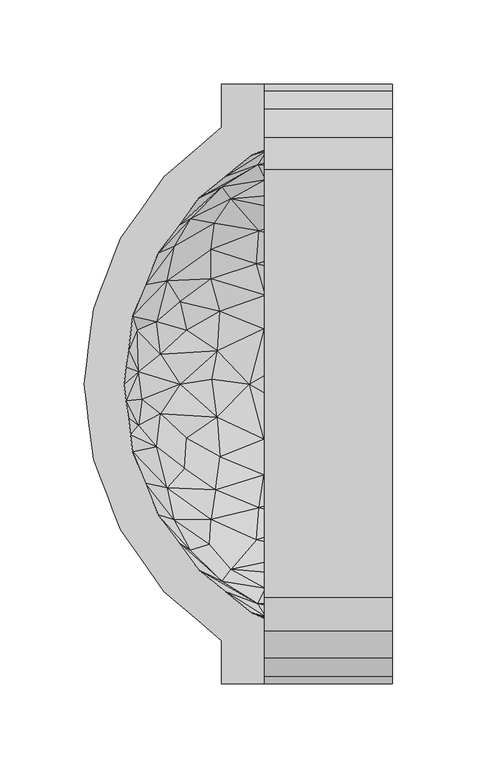
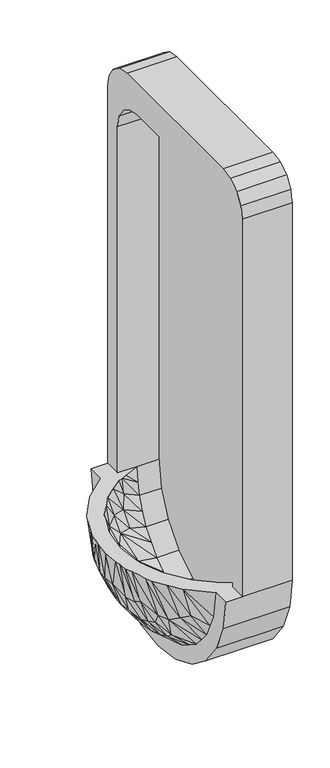
"""IFC4 building model written with IfcOpenShell, lengths in millimetres: proxy geometry, Urinal-Wall-3D:Urinal-Wall-3D:2445:Urinal-Wall-3D:2445 : Urinal-Wall-3D:Urinal-Wall-3D:2445:300497 : Urinal-Wall-3D:Urinal-Wall-3D:2445:Urinal-Wall-3D:2445 : Urinal-Wall-3D:Urinal-Wall-3D:2445:300497."""

from ifc_helpers import new_model, si_unit, origin, place, context, project, spatial, triangles, source, transform, mapped, element, save


def generic_models_a574338b(model_context):
    return source(origin(), model_context, "Body", "Tessellation", [
        triangles([(647621.4931641, -572395.2011719, 609.6), (647612.1914062, -572368.1144531, 609.6), (647599.2433594, -572386.4575195, 609.6), (647595.1505859, -572396.9499023, 609.6), (647645.0824219, -572332.5817383, 609.6), (647625.0650391, -572349.7713867, 609.6), (647645.5289063, -572362.6450195, 609.6), (647633.4738281, -572378.9044922, 609.6), (647613.9029297, -572413.9907227, 609.6), (647587.1138672, -572417.8602539, 609.6), (647606.3871094, -572432.7430664, 609.6), (647591.1322266, -572407.4050781, 609.6), (647581.6816406, -572439.4775391, 609.6), (647583.0210938, -572428.3526367, 609.6), (647603.8570313, -572452.8348633, 609.6), (647580.2677734, -572450.6024414, 609.6), (647602.5175781, -572462.8435547, 609.6), (647578.9283203, -572461.7645508, 609.6), (647684.521875, -572295.0770508, 609.6), (647659.1466797, -572295.0770508, 609.6), (647684.521875, -572320.4894531, 609.6), (647659.1466797, -572320.4894531, 609.6), (647677.0060547, -572337.1954102, 609.6), (647661.2302734, -572349.9202148, 609.6), (647713.8410156, -572320.4894531, 609.6), (647690.8470703, -572330.9446289, 609.6), (647683.9265625, -572334.0700195, 609.6), (647605.1220703, -572442.7889648, 609.6), (647601.2525391, -572472.8894531, 609.6), (647577.5144531, -572472.8894531, 609.6), (647578.9283203, -572484.0143555, 609.6), (647580.2677734, -572495.1764648, 609.6), (647602.5175781, -572482.9353516, 609.6), (647603.8570313, -572492.944043, 609.6), (647605.1220703, -572502.9899414, 609.6), (647581.6816406, -572506.3013672, 609.6), (647606.3871094, -572513.0358398, 609.6), (647583.0210938, -572517.4262695, 609.6), (647587.1138672, -572527.9186523, 609.6), (647613.9029297, -572531.8253906, 609.6), (647591.1322266, -572538.3738281, 609.6), (647595.1505859, -572548.8662109, 609.6), (647621.4931641, -572550.5777344, 609.6), (647599.2433594, -572559.3213867, 609.6), (647612.1914062, -572577.6644531, 609.6), (647633.4738281, -572566.8744141, 609.6), (647645.5289063, -572583.1338867, 609.6), (647625.0650391, -572596.0075195, 609.6), (647661.2302734, -572595.8586914, 609.6), (647645.0824219, -572613.197168, 609.6), (647690.8470703, -572614.8342773, 609.6), (647677.0060547, -572608.5834961, 609.6), (647684.521875, -572625.2894531, 609.6), (647659.1466797, -572625.2894531, 609.6), (647659.1466797, -572650.7018555, 609.6), (647702.3068359, -572620.0804687, 609.6), (647713.8410156, -572625.2894531, 609.6), (647684.521875, -572650.7018555, 609.6), (647685.8613281, -572334.4420898, 583.9469873), (647659.2955078, -572589.8683594, 571.4722764), (647713.8410156, -572391.3316406, 482.6979349), (647713.8410156, -572373.1001953, 494.4237817), (647681.3220703, -572381.9182617, 505.4282335), (647664.8765625, -572582.7618164, 545.0935813), (647685.1171875, -572594.184375, 538.9458097), (647713.8410156, -572586.8917969, 510.8150414), (647609.8101563, -572465.6712891, 558.6713862), (647664.8765625, -572363.0170898, 545.0936176), (647713.8410156, -572358.8871094, 510.8150414), (647685.1171875, -572351.5945313, 538.9458097), (647713.8410156, -572554.4472656, 482.6979349), (647679.8337891, -572565.3117188, 507.9383274), (647713.8410156, -572572.6787109, 494.4237817), (647684.4474609, -572440.1472656, 473.4506433), (647685.3404297, -572420.0182617, 479.4091822), (647658.1792969, -572429.7292969, 495.410422), (647656.6166016, -572453.2069336, 490.4112722), (647675.5921875, -572472.8894531, 474.7844645), (647713.8410156, -572326.6658203, 566.663958), (647713.8410156, -572323.8380859, 586.2369638), (647680.6523438, -572342.5904297, 564.4870923), (647659.2955078, -572355.9105469, 571.4722764), (647638.3851562, -572440.9658203, 512.4167241), (647622.9070313, -572455.2533203, 531.3763953), (647638.3851562, -572504.8875, 512.4541128), (647622.9070313, -572490.3767578, 531.3513605), (647620.6746094, -572509.9848633, 543.0548249), (647679.8337891, -572401.4519531, 492.2453536), (647658.1792969, -572516.0496094, 495.410422), (647684.4474609, -572526.5791992, 480.2694131), (647684.3730469, -572505.5572266, 473.4754601), (647630.7949219, -572553.4426758, 564.2788201), (647626.7021484, -572534.3182617, 548.7818009), (647640.8408203, -572374.8117188, 571.7064554), (647637.1945313, -572522.8584961, 522.0602489), (647685.8613281, -572611.3368164, 583.9469873), (647680.6523438, -572603.1884766, 564.4870923), (647713.8410156, -572344.6740234, 527.2063374), (647713.8410156, -572335.6699219, 546.9351477), (647652.0773438, -572568.027832, 542.0659318), (647655.0539063, -572377.3045898, 538.0613434), (647652.7470703, -572392.8199219, 523.79539), (647713.8410156, -572610.1089844, 546.9351477), (647681.3220703, -572546.1500977, 492.3042526), (647713.8410156, -572536.2158203, 470.9720881), (647609.8845703, -572497.2600586, 563.910783), (647608.9916016, -572440.9658203, 572.3650998), (647631.1669922, -572391.2200195, 565.2611003), (647626.7021484, -572411.4606445, 548.7818009), (647713.8410156, -572619.1130859, 566.663958), (647713.8410156, -572623.6151367, 597.9184819), (647713.8410156, -572621.9408203, 586.2369638), (647713.8410156, -572409.600293, 470.9720881), (647640.5431641, -572571.4136719, 573.9630401), (647655.4259766, -572535.7321289, 507.6571309), (647713.8410156, -572451.1977539, 458.7512135), (647713.8410156, -572472.8894531, 458.7512135), (647713.8410156, -572494.5811523, 458.7512135), (647713.8410156, -572601.1048828, 527.2063374), (647620.6746094, -572435.794043, 543.0548249), (647713.8410156, -572430.3990234, 464.8616326), (647611.89375, -572481.9679688, 553.1137676), (647634.4412109, -572472.8894531, 512.2263288), (647656.4677734, -572492.5347656, 490.5842631), (647634.5900391, -572423.887793, 525.2664122), (647652.7470703, -572552.9589844, 523.79539), (647652.7470703, -572410.4188477, 510.2499232), (647653.3423828, -572469.9873047, 491.7342293), (647713.8410156, -572515.3798828, 464.8616326), (647747.9970703, -572326.6658203, 566.663958), (647747.9970703, -572320.4894531, 609.6), (647747.9970703, -572344.6740234, 527.2063374), (647747.9970703, -572409.600293, 470.9720881), (647747.9970703, -572373.1001953, 494.4237817), (647747.9970703, -572451.1977539, 458.7512135), (647747.9970703, -572494.5811523, 458.7512135), (647747.9970703, -572536.2158203, 470.9720881), (647747.9970703, -572572.6787109, 494.4237817), (647747.9970703, -572625.2894531, 609.6), (647747.9970703, -572619.1130859, 566.663958), (647747.9970703, -572601.1048828, 527.2063374), (647760.721875, -572609.625293, 1268.066494), (647760.721875, -572619.3363281, 1266.1330364), (647760.721875, -572627.559082, 1260.6271225), (647760.721875, -572648.7670898, 1228.9201916), (647760.721875, -572599.8770508, 1269.9999516), (647760.721875, -572641.3256836, 1246.8807232), (647760.721875, -572635.819043, 1255.1210632), (647760.721875, -572295.0770508, 1219.2), (647760.721875, -572345.9018555, 1269.9999516), (647760.721875, -572318.2198242, 1260.6271225), (647760.721875, -572336.1536133, 1268.066494), (647760.721875, -572304.4532227, 1246.8807232), (647760.721875, -572326.4425781, 1266.1330364), (647760.721875, -572297.0118164, 1228.9201916), (647760.721875, -572309.9598633, 1255.1210632), (647760.721875, -572298.946582, 1238.6403831), (647760.721875, -572646.8323242, 1238.6403831), (647760.721875, -572650.7018555, 1219.2), (647760.721875, -572644.6371094, 563.5819877), (647760.721875, -572295.0770508, 609.6), (647760.721875, -572650.7018555, 609.6), (647760.721875, -572318.9267578, 520.7000121), (647760.721875, -572626.8521484, 520.7000121), (647760.721875, -572598.6120117, 483.876424), (647760.721875, -572561.7770508, 455.6206996), (647760.721875, -572347.1668945, 483.876424), (647760.721875, -572301.1417969, 563.5819877), (647760.721875, -572518.9145508, 437.8583754), (647760.721875, -572384.0018555, 455.6206996), (647760.721875, -572426.8643555, 437.8583754), (647760.721875, -572472.8894531, 431.7999879), (647659.1466797, -572301.1417969, 563.5819877), (647659.1466797, -572347.1668945, 483.876424), (647659.1466797, -572318.9267578, 520.7000121), (647659.1466797, -572384.0018555, 455.6206996), (647659.1466797, -572426.8643555, 437.8583754), (647659.1466797, -572472.8894531, 431.7999879), (647659.1466797, -572518.9145508, 437.8583754), (647659.1466797, -572561.7770508, 455.6206996), (647659.1466797, -572626.8521484, 520.7000121), (647659.1466797, -572644.6371094, 563.5819877), (647659.1466797, -572598.6120117, 483.876424), (647659.1466797, -572472.8894531, 458.7512135), (647659.1466797, -572494.5811523, 458.7512135), (647659.1466797, -572451.1977539, 458.7512135), (647659.1466797, -572554.4472656, 482.6979349), (647659.1466797, -572536.2158203, 470.9720881), (647659.1466797, -572572.6787109, 494.4237817), (647659.1466797, -572515.3798828, 464.8616326), (647659.1466797, -572430.3990234, 464.8616326), (647659.1466797, -572409.600293, 470.9720881), (647659.1466797, -572391.3316406, 482.6979349), (647659.1466797, -572373.1001953, 494.4237817), (647659.1466797, -572358.8871094, 510.8150414), (647659.1466797, -572344.6740234, 527.2063374), (647659.1466797, -572610.1089844, 546.9351477), (647659.1466797, -572601.1048828, 527.2063374), (647659.1466797, -572586.8917969, 510.8150414), (647659.1466797, -572622.2384766, 588.2859303), (647659.1466797, -572619.1130859, 566.663958), (647659.1466797, -572335.6699219, 546.9351477), (647659.1466797, -572326.6658203, 566.663958), (647659.1466797, -572323.5404297, 588.2859303), (647636.5248047, -572400.1869141, 496.2975772), (647629.2322266, -572417.971875, 494.5229762), (647612.3402344, -572400.6333984, 530.1853706), (647635.7806641, -572346.7204102, 564.7131323), (647606.6847656, -572415.1069336, 529.1428834), (647627.5207031, -572385.5645508, 519.1144621), (647604.6011719, -572392.3734375, 557.7764917), (647618.7398438, -572375.3326172, 547.3545261), (647626.8509766, -572359.4080078, 557.2311399), (647630.94375, -572505.4828125, 484.5077808), (647630.94375, -572440.2960938, 484.5077808), (647594.9273438, -572409.7863281, 563.8420009), (647606.9080078, -572449.9699219, 512.8612101), (647585.4767578, -572457.7833984, 558.5052627), (647589.4951172, -572439.4775391, 553.8611421), (647626.8509766, -572586.3708984, 557.2311399), (647635.7806641, -572599.0584961, 564.7131323), (647630.94375, -572526.1699219, 491.8173274), (647607.9498047, -572515.3054688, 517.92133), (647612.3402344, -572545.1455078, 530.1853706), (647633.1761719, -572541.1643555, 497.2734624), (647631.6134766, -572554.89375, 508.7941981), (647592.9925781, -572524.4956055, 557.1740939), (647589.1230469, -572508.1245117, 555.9720234), (647625.7347656, -572485.5398438, 486.402905), (647600.8804688, -572494.9160156, 522.8274985), (647602.0710938, -572472.8894531, 518.0100964), (647627.7439453, -572462.6947266, 484.0731417), (647583.7652344, -572482.5632813, 563.1875713), (647607.9498047, -572430.4734375, 517.92133), (647590.4625, -572422.4367188, 564.5393057), (647609.4380859, -572556.9029297, 549.5402212), (647594.8529297, -572536.1786133, 564.3948741), (647618.7398438, -572570.4462891, 547.3544898), (647609.8845703, -572529.9650391, 522.8140182), (647684.521875, -572625.2894531, 1168.3999758), (647684.521875, -572623.6151367, 1176.8655928), (647684.521875, -572650.7018555, 1219.2), (647684.521875, -572621.4199219, 1187.8402863), (647684.521875, -572610.4066406, 1204.321039), (647684.521875, -572615.9132813, 1196.080699), (647684.521875, -572627.559082, 1260.6271225), (647684.521875, -572593.9239258, 1215.3330849), (647684.521875, -572602.1838867, 1209.8270256), (647684.521875, -572584.2128906, 1217.2665424), (647684.521875, -572599.8770508, 1269.9999516), (647684.521875, -572641.3256836, 1246.8807232), (647684.521875, -572322.4242187, 1178.1201674), (647684.521875, -572324.3589844, 1187.8402863), (647684.521875, -572295.0770508, 1219.2), (647684.521875, -572320.4894531, 1168.3999758), (647684.521875, -572351.8549805, 1215.3330849), (647684.521875, -572362.8310547, 1217.5160912), (647684.521875, -572345.9018555, 1269.9999516), (647684.521875, -572304.4532227, 1246.8807232), (647684.521875, -572335.3722656, 1204.321039), (647684.521875, -572343.5950195, 1209.8270256), (647684.521875, -572329.865625, 1196.080699), (647684.521875, -572318.2198242, 1260.6271225), (647684.521875, -572648.7670898, 1228.9201916), (647684.521875, -572646.8323242, 1238.6403831), (647684.521875, -572619.3363281, 1266.1330364), (647684.521875, -572606.9463867, 1268.5966942), (647684.521875, -572574.5018555, 1219.2), (647684.521875, -572635.819043, 1255.1210632), (647684.521875, -572371.2770508, 1219.2), (647684.521875, -572298.946582, 1238.6403831), (647684.521875, -572296.490918, 1226.2546566), (647684.521875, -572336.1536133, 1268.066494), (647684.521875, -572309.9598633, 1255.1210632), (647684.521875, -572326.4425781, 1266.1330364), (647747.9970703, -572320.4894531, 1168.3999758), (647747.9970703, -572324.3589844, 1187.8402863), (647747.9970703, -572322.1637695, 1176.8655928), (647747.9970703, -572335.3722656, 1204.321039), (647747.9970703, -572329.865625, 1196.080699), (647747.9970703, -572351.8549805, 1215.3330849), (647747.9970703, -572361.5660156, 1217.2665424), (647747.9970703, -572371.2770508, 1219.2), (647747.9970703, -572343.5950195, 1209.8270256), (647747.9970703, -572574.5018555, 1219.2), (647747.9970703, -572593.9239258, 1215.3330849), (647747.9970703, -572582.9478516, 1217.5160912), (647747.9970703, -572610.4066406, 1204.321039), (647747.9970703, -572602.1838867, 1209.8270256), (647747.9970703, -572621.4199219, 1187.8402863), (647747.9970703, -572623.3546875, 1178.1201674), (647747.9970703, -572625.2894531, 1168.3999758), (647747.9970703, -572615.9132813, 1196.080699)], [[1, 2, 3], [1, 3, 4], [5, 6, 7], [2, 8, 6], [1, 8, 2], [4, 9, 1], [9, 10, 11], [9, 12, 10], [13, 11, 14], [10, 14, 11], [15, 13, 16], [17, 16, 18], [12, 9, 4], [19, 20, 21], [21, 20, 22], [23, 22, 24], [21, 22, 23], [25, 21, 26], [27, 26, 21], [21, 23, 27], [7, 6, 8], [15, 28, 13], [11, 13, 28], [24, 22, 5], [17, 15, 16], [17, 18, 29], [24, 5, 7], [18, 30, 29], [31, 32, 33], [31, 33, 29], [33, 32, 34], [36, 35, 34], [35, 36, 37], [36, 34, 32], [31, 29, 30], [38, 39, 37], [37, 39, 40], [40, 41, 42], [39, 41, 40], [40, 42, 43], [43, 42, 44], [38, 37, 36], [43, 45, 46], [45, 43, 44], [47, 46, 48], [49, 47, 50], [51, 52, 53], [49, 54, 52], [45, 48, 46], [49, 50, 54], [54, 55, 53], [54, 53, 52], [57, 56, 53], [58, 53, 55], [56, 51, 53], [50, 47, 48], [59, 23, 24], [46, 47, 60], [61, 62, 63], [64, 65, 66], [29, 67, 17], [15, 17, 67], [68, 69, 70], [71, 72, 73], [74, 75, 76], [74, 77, 78], [79, 80, 27], [80, 26, 27], [25, 26, 80], [70, 81, 82], [7, 81, 24], [77, 83, 84], [85, 86, 87], [61, 63, 88], [89, 90, 91], [40, 92, 93], [94, 8, 1], [89, 85, 95], [96, 49, 52], [97, 60, 47], [7, 82, 81], [81, 98, 99], [72, 100, 64], [63, 101, 102], [96, 103, 97], [71, 104, 72], [71, 105, 104], [86, 106, 87], [15, 107, 28], [11, 28, 107], [108, 109, 102], [52, 110, 96], [56, 57, 111], [51, 56, 112], [52, 112, 110], [52, 51, 112], [112, 56, 111], [113, 61, 88], [64, 100, 114], [90, 89, 115], [79, 27, 59], [116, 78, 117], [118, 117, 78], [47, 49, 97], [8, 94, 82], [60, 65, 64], [8, 82, 7], [70, 82, 68], [119, 65, 97], [81, 70, 98], [62, 69, 68], [69, 98, 70], [114, 60, 64], [60, 97, 65], [64, 66, 73], [65, 119, 66], [109, 11, 120], [59, 99, 79], [97, 103, 119], [121, 75, 74], [33, 106, 122], [84, 83, 120], [87, 106, 35], [123, 122, 86], [85, 89, 124], [120, 83, 125], [92, 43, 114], [102, 101, 108], [109, 9, 11], [93, 126, 115], [93, 37, 40], [24, 81, 59], [99, 59, 81], [103, 96, 110], [97, 49, 96], [59, 27, 23], [74, 116, 121], [91, 124, 89], [102, 88, 63], [62, 68, 63], [68, 101, 63], [102, 127, 88], [127, 76, 75], [68, 94, 101], [108, 1, 9], [108, 101, 94], [109, 108, 9], [127, 102, 109], [125, 109, 120], [77, 74, 76], [88, 75, 113], [78, 116, 74], [83, 77, 76], [128, 78, 77], [113, 75, 121], [75, 88, 127], [94, 68, 82], [108, 94, 1], [76, 127, 125], [107, 84, 120], [67, 123, 84], [77, 84, 123], [76, 125, 83], [127, 109, 125], [104, 115, 126], [104, 105, 90], [104, 126, 72], [100, 72, 126], [64, 73, 72], [92, 100, 126], [100, 92, 114], [93, 92, 126], [40, 43, 92], [91, 129, 118], [129, 91, 90], [118, 78, 91], [124, 91, 78], [128, 124, 78], [86, 85, 124], [90, 105, 129], [90, 115, 104], [115, 89, 95], [43, 46, 114], [60, 114, 46], [86, 124, 123], [95, 87, 93], [67, 122, 123], [33, 34, 106], [35, 106, 34], [87, 95, 85], [115, 95, 93], [86, 122, 106], [35, 37, 87], [67, 29, 33], [37, 93, 87], [33, 122, 67], [107, 67, 84], [77, 123, 128], [11, 107, 120], [15, 67, 107], [124, 128, 123], [79, 130, 80], [80, 131, 25], [131, 80, 130], [132, 130, 99], [79, 99, 130], [99, 98, 132], [113, 133, 61], [61, 134, 62], [134, 61, 133], [62, 134, 69], [69, 132, 98], [132, 69, 134], [116, 135, 121], [121, 133, 113], [133, 121, 135], [135, 116, 117], [117, 118, 136], [117, 136, 135], [137, 105, 71], [71, 73, 138], [71, 138, 137], [136, 118, 129], [129, 105, 137], [129, 137, 136], [111, 57, 139], [112, 139, 140], [139, 112, 111], [112, 140, 110], [103, 140, 141], [140, 103, 110], [103, 141, 119], [66, 141, 138], [141, 66, 119], [66, 138, 73], [142, 143, 144], [145, 146, 142], [142, 147, 145], [144, 148, 147], [142, 144, 147], [149, 150, 146], [153, 151, 152], [151, 154, 152], [155, 152, 150], [153, 156, 151], [155, 157, 153], [152, 155, 153], [149, 155, 150], [145, 147, 158], [149, 146, 159], [162, 160, 161], [149, 159, 162], [163, 164, 165], [165, 166, 167], [160, 164, 168], [166, 169, 170], [164, 163, 168], [160, 168, 161], [161, 149, 162], [169, 171, 170], [167, 166, 170], [165, 167, 163], [171, 169, 172], [159, 146, 145], [19, 168, 173], [168, 19, 161], [19, 173, 20], [174, 175, 167], [163, 167, 175], [176, 174, 170], [167, 170, 174], [173, 168, 163], [163, 175, 173], [177, 176, 171], [170, 171, 176], [178, 177, 172], [171, 172, 177], [169, 179, 172], [178, 172, 179], [169, 166, 180], [180, 179, 169], [181, 164, 182], [160, 182, 164], [164, 181, 165], [183, 165, 181], [165, 183, 166], [180, 166, 183], [160, 162, 58], [58, 55, 182], [58, 182, 160], [184, 178, 185], [184, 186, 178], [178, 179, 185], [178, 186, 177], [180, 187, 188], [189, 187, 180], [190, 185, 179], [179, 188, 190], [179, 180, 188], [177, 191, 192], [191, 177, 186], [176, 192, 193], [192, 176, 177], [194, 174, 176], [174, 195, 175], [195, 174, 194], [195, 196, 175], [194, 176, 193], [181, 197, 198], [197, 181, 182], [199, 181, 198], [181, 199, 183], [182, 55, 200], [182, 200, 201], [200, 55, 54], [182, 201, 197], [199, 189, 183], [202, 173, 175], [203, 204, 173], [204, 20, 173], [20, 204, 22], [202, 203, 173], [202, 175, 196], [189, 180, 183], [6, 5, 204], [6, 204, 203], [22, 204, 5], [205, 206, 207], [208, 202, 196], [206, 209, 207], [210, 211, 212], [3, 2, 213], [214, 185, 190], [6, 202, 208], [191, 215, 206], [213, 212, 3], [6, 203, 202], [205, 207, 210], [211, 216, 10], [217, 218, 219], [220, 221, 45], [197, 201, 48], [214, 222, 223], [201, 200, 48], [200, 50, 48], [54, 50, 200], [2, 208, 213], [224, 225, 226], [227, 36, 228], [229, 230, 231], [198, 197, 221], [205, 193, 192], [221, 48, 45], [232, 229, 231], [221, 220, 198], [233, 231, 230], [219, 218, 16], [215, 217, 234], [234, 235, 209], [217, 215, 232], [224, 236, 237], [227, 237, 38], [189, 238, 226], [208, 196, 213], [2, 6, 208], [212, 195, 194], [195, 212, 213], [193, 210, 194], [212, 211, 4], [213, 196, 195], [48, 221, 197], [220, 45, 44], [238, 220, 44], [238, 199, 220], [236, 42, 41], [236, 41, 39], [187, 226, 225], [189, 199, 238], [199, 198, 220], [226, 236, 224], [206, 205, 192], [210, 207, 211], [215, 234, 206], [206, 234, 209], [194, 210, 212], [193, 205, 210], [206, 192, 191], [232, 215, 186], [191, 186, 215], [229, 184, 185], [184, 229, 232], [232, 231, 217], [217, 231, 218], [233, 218, 231], [16, 218, 18], [30, 18, 218], [229, 185, 214], [214, 230, 229], [223, 228, 230], [30, 233, 31], [32, 31, 233], [233, 230, 228], [218, 233, 30], [232, 186, 184], [227, 228, 223], [32, 233, 228], [223, 222, 239], [228, 36, 32], [227, 38, 36], [190, 188, 222], [188, 225, 222], [223, 239, 227], [222, 214, 190], [214, 223, 230], [234, 219, 235], [216, 207, 209], [219, 16, 13], [10, 12, 211], [12, 4, 211], [216, 14, 10], [216, 211, 207], [238, 44, 42], [239, 237, 227], [187, 225, 188], [236, 39, 237], [237, 39, 38], [239, 225, 224], [189, 226, 187], [236, 226, 238], [42, 236, 238], [216, 235, 14], [217, 219, 234], [13, 14, 235], [209, 235, 216], [219, 13, 235], [225, 239, 222], [237, 239, 224], [4, 3, 212], [53, 58, 240], [242, 241, 240], [242, 243, 241], [58, 242, 240], [242, 244, 245], [246, 247, 248], [249, 247, 250], [248, 244, 251], [245, 243, 242], [252, 253, 254], [19, 21, 255], [19, 255, 254], [255, 252, 254], [256, 257, 258], [259, 260, 261], [253, 262, 254], [261, 256, 263], [254, 262, 260], [251, 244, 264], [246, 248, 251], [251, 264, 265], [266, 247, 246], [264, 244, 242], [250, 247, 267], [268, 249, 250], [266, 267, 247], [251, 269, 246], [270, 268, 250], [259, 271, 260], [261, 263, 259], [272, 254, 260], [260, 271, 272], [258, 257, 270], [256, 273, 263], [263, 274, 259], [273, 275, 263], [256, 258, 273], [258, 270, 250], [276, 255, 25], [21, 25, 255], [25, 131, 276], [277, 253, 252], [277, 252, 278], [278, 255, 276], [255, 278, 252], [279, 260, 262], [279, 262, 280], [262, 277, 280], [277, 262, 253], [256, 281, 282], [256, 282, 257], [257, 283, 270], [283, 257, 282], [260, 279, 284], [260, 284, 261], [284, 256, 261], [256, 284, 281], [285, 268, 270], [270, 283, 285], [286, 247, 249], [286, 249, 287], [287, 268, 285], [268, 287, 249], [288, 244, 248], [288, 248, 289], [248, 286, 289], [286, 248, 247], [243, 290, 291], [243, 291, 241], [241, 292, 240], [292, 241, 291], [244, 288, 293], [244, 293, 245], [293, 243, 245], [243, 293, 290], [57, 240, 292], [240, 57, 53], [57, 292, 139], [159, 242, 162], [58, 162, 242], [148, 269, 251], [148, 251, 147], [251, 158, 147], [158, 251, 265], [242, 159, 145], [242, 145, 264], [145, 265, 264], [265, 145, 158], [146, 250, 267], [146, 267, 142], [142, 266, 143], [266, 142, 267], [246, 269, 148], [266, 246, 143], [148, 144, 246], [144, 143, 246], [150, 258, 250], [250, 146, 150], [156, 274, 263], [156, 263, 151], [263, 154, 151], [154, 263, 275], [258, 150, 152], [258, 152, 273], [152, 275, 273], [275, 152, 154], [149, 254, 272], [149, 272, 155], [155, 271, 157], [271, 155, 272], [259, 274, 156], [271, 259, 157], [156, 153, 259], [153, 157, 259], [161, 19, 149], [254, 149, 19], [292, 285, 276], [283, 282, 278], [282, 284, 280], [284, 279, 280], [284, 282, 281], [285, 283, 276], [293, 288, 289], [291, 290, 293], [291, 293, 289], [287, 291, 289], [292, 291, 287], [292, 287, 285], [287, 289, 286], [278, 282, 280], [283, 278, 276], [139, 292, 276], [140, 131, 130], [130, 132, 141], [276, 131, 139], [132, 134, 138], [130, 141, 140], [132, 138, 141], [139, 131, 140], [133, 135, 136], [133, 136, 137], [134, 137, 138], [134, 133, 137], [278, 280, 277]]),
    ])


if __name__ == "__main__":
    model = new_model("IFC4")
    model_context = context("Model", 3, world=origin())
    ifc_project = project(units=[si_unit("LENGTHUNIT", "METRE", prefix="MILLI")], contexts=[model_context])
    site = spatial("IfcSite", under=ifc_project)
    building = spatial("IfcBuilding", under=site)
    placement = place(None, origin())
    generic_models_shape = generic_models_a574338b(model_context)
    element("IfcBuildingElementProxy", 1, Name="Urinal-Wall-3D:Urinal-Wall-3D:2445:Urinal-Wall-3D:2445 : Urinal-Wall-3D:Urinal-Wall-3D:2445:300497 : Urinal-Wall-3D:Urinal-Wall-3D:2445:Urinal-Wall-3D:2445 : Urinal-Wall-3D:Urinal-Wall-3D:2445:300497", ObjectType="Urinal-Wall-3D:Urinal-Wall-3D:2445:Urinal-Wall-3D:2445 : Urinal-Wall-3D:Urinal-Wall-3D:2445:300497 : Urinal-Wall-3D:Urinal-Wall-3D:2445:Urinal-Wall-3D:2445 : Urinal-Wall-3D:Urinal-Wall-3D:2445:300497", at=placement, inside=building, context=model_context, shape_type="MappedRepresentation", body=[
        mapped(generic_models_shape, transform((0.0, 0.0, 0.0), x_axis=(1.0, 0.0, 0.0), y_axis=(0.0, 1.0, 0.0), z_axis=(0.0, 0.0, 1.0))),
    ])
    save(model, "model.ifc")

# Revit data of these elements
# Type "Urinal-Wall-3D:Urinal-Wall-3D:2445:Urinal-Wall-3D:2445 : Urinal-Wall-3D:Urinal-Wall-3D:2445:300497 : Urinal-Wall-3D:Urinal-Wall-3D:2445:Urinal-Wall-3D:2445 : Urinal-Wall-3D:Urinal-Wall-3D:2445:300497"
#   NameOverride = "Urinal-Wall-3D:Urinal-Wall-3D:2445:Urinal-Wall-3D:2445 : Urinal-Wall-3D:Urinal-Wall-3D:2445:300497"
#   ObjectTypeOverride = "Urinal-Wall-3D:2445 : Urinal-Wall-3D:Urinal-Wall-3D:2445"
#   Tag = "300497"
#   Reference = "Urinal-Wall-3D"
